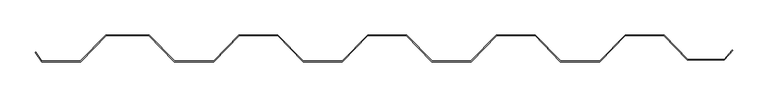
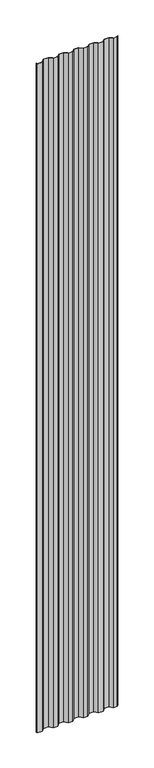
"""IFC4 building model written with IfcOpenShell, lengths in millimetres: proxy geometry, Generic Models 2:Generic Models 2:310765:Generic Models 2:310765 : Generic Models 2:Generic Models 2:310765:90 : Generic Models 2:Generic Models 2:310765:Generic Models 2:310765 : Generic Models 2:Generic Models 2:310765:300385."""

from ifc_helpers import new_model, si_unit, origin, origin_with_axes, place, context, project, spatial, polyline, outline, extrude, source, transform, mapped, element, save


def generic_models_fad994c5(model_context):
    return source(origin(), model_context, "Body", "SweptSolid", [
        extrude(outline(polyline([(593719.8809779, -536567.1923731), (593667.2871722, -536567.1923731), (593633.6551875, -536532.6342858), (593579.1467875, -536532.6342858), (593542.9845958, -536569.9405358), (593486.9373791, -536569.9405358), (593450.7751875, -536532.6342858), (593396.2667875, -536532.6342858), (593360.1045958, -536569.9405358), (593304.0573791, -536569.9405358), (593267.8951875, -536532.6342858), (593213.3867875, -536532.6342858), (593177.2245958, -536569.9405358), (593121.1773791, -536569.9405358), (593085.0151875, -536532.6342858), (593030.5067875, -536532.6342858), (592994.3445958, -536569.9405358), (592938.2973791, -536569.9405358), (592902.1351875, -536532.6342858), (592841.2767875, -536532.6342858), (592805.1145958, -536569.9405358), (592749.8367875, -536569.9405358), (592740.6584173, -536556.8324648), (592741.3086193, -536556.3771885), (592750.2499875, -536569.1467858), (592804.7785503, -536569.1467858), (592840.9407419, -536531.8405358), (592902.471233, -536531.8405358), (592938.6334246, -536569.1467858), (592994.0085503, -536569.1467858), (593030.1707419, -536531.8405358), (593085.351233, -536531.8405358), (593121.5134246, -536569.1467858), (593176.8885503, -536569.1467858), (593213.0507419, -536531.8405358), (593268.231233, -536531.8405358), (593304.3934246, -536569.1467858), (593359.7685503, -536569.1467858), (593395.9307419, -536531.8405358), (593451.111233, -536531.8405358), (593487.2734246, -536569.1467858), (593542.6485503, -536569.1467858), (593578.8107419, -536531.8405358), (593633.9903018, -536531.8405358), (593667.6222866, -536566.3986231), (593719.5286406, -536566.3986231), (593731.1747524, -536553.5223302), (593731.7367242, -536554.084302), (593719.8809779, -536567.1923731)])), origin_with_axes(), (0.0, 0.0, 1.0), 8564.7690068),
    ])


if __name__ == "__main__":
    model = new_model("IFC4")
    model_context = context("Model", 3, world=origin())
    ifc_project = project(units=[si_unit("LENGTHUNIT", "METRE", prefix="MILLI")], contexts=[model_context])
    site = spatial("IfcSite", under=ifc_project)
    building = spatial("IfcBuilding", under=site)
    placement = place(None, origin())
    generic_models_shape = generic_models_fad994c5(model_context)
    element("IfcBuildingElementProxy", 1, Name="Generic Models 2:Generic Models 2:310765:Generic Models 2:310765 : Generic Models 2:Generic Models 2:310765:90 : Generic Models 2:Generic Models 2:310765:Generic Models 2:310765 : Generic Models 2:Generic Models 2:310765:300385", ObjectType="Generic Models 2:Generic Models 2:310765:Generic Models 2:310765 : Generic Models 2:Generic Models 2:310765:90 : Generic Models 2:Generic Models 2:310765:Generic Models 2:310765 : Generic Models 2:Generic Models 2:310765:300385", at=placement, inside=building, context=model_context, shape_type="MappedRepresentation", body=[
        mapped(generic_models_shape, transform((0.0, 0.0, 0.0), x_axis=(1.0, 0.0, 0.0), y_axis=(0.0, 1.0, 0.0), z_axis=(0.0, 0.0, 1.0))),
    ])
    save(model, "model.ifc")

# Revit data of these elements
# Type "Generic Models 2:Generic Models 2:310765:Generic Models 2:310765 : Generic Models 2:Generic Models 2:310765:90 : Generic Models 2:Generic Models 2:310765:Generic Models 2:310765 : Generic Models 2:Generic Models 2:310765:300385"
#   NameOverride = "Generic Models 2:Generic Models 2:310765:Generic Models 2:310765 : Generic Models 2:Generic Models 2:310765:300385"
#   ObjectTypeOverride = "Generic Models 2:310765 : Generic Models 2:Generic Models 2:310765"
#   Reference = "Generic Models 2"
#   Tag = "300385"
# Element 1 (IfcBuildingElementProxy, "Generic Models 2:Generic Models 2:310765:Generic Models 2:310765 : Generic Models 2:Generic Models 2:310765:90 : Generic Models 2:Generic Models 2:310765:Generic Models 2:310765 : Generic Models 2:Generic Models 2:310765:300385")
#   Materials on its faces: "VERTICAL CORRUGATED METAL PANEL - EXPOSED FASTENERS - (MBCI 7.2 PANEL)"
# Materials
#   "VERTICAL CORRUGATED METAL PANEL - EXPOSED FASTENERS - (MBCI 7.2 PANEL)": class "Generic", colour RGB 120 120 120, transparency 0, Cost = 0
